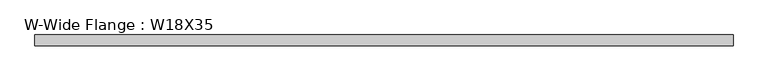
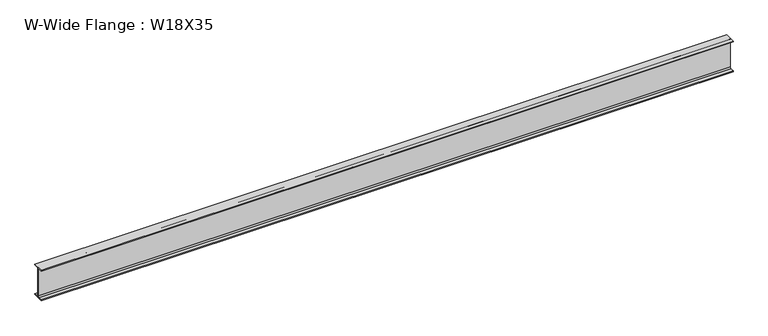
"""IFC4 building model written with IfcOpenShell, lengths in millimetres: beam geometry, W-Wide Flange : W18X35."""

from ifc_helpers import new_model, si_unit, point, frame, frame_2d, origin, place, context, project, spatial, polyline, circle_curve, trimmed, segment, composite_curve, outline, extrude, source, transform, mapped, element, save


def w_wide_flange_w18x35_eb31aa4e(model_context):
    return source(origin(), model_context, "Body", "SweptSolid", [
        extrude(outline(composite_curve([segment(polyline([(76.2, -213.995), (76.2, -224.79), (-76.2, -224.79), (-76.2, -213.995), (-21.59, -213.995)]), True, "CONTINUOUS"), segment(trimmed(circle_curve(frame_2d((-21.59, -196.215)), 17.78), [point((-21.59, -213.995))], [point((-3.81, -196.215))], True, "CARTESIAN"), True, "CONTINUOUS"), segment(polyline([(-3.81, -196.215), (-3.81, 196.215)]), True, "CONTINUOUS"), segment(trimmed(circle_curve(frame_2d((-21.59, 196.215)), 17.78), [point((-3.81, 196.215))], [point((-21.59, 213.995))], True, "CARTESIAN"), True, "CONTINUOUS"), segment(polyline([(-21.59, 213.995), (-76.2, 213.995), (-76.2, 224.79), (76.2, 224.79), (76.2, 213.995), (21.59, 213.995)]), True, "CONTINUOUS"), segment(trimmed(circle_curve(frame_2d((21.59, 196.215)), 17.78), [point((21.59, 213.995))], [point((3.81, 196.215))], True, "CARTESIAN"), True, "CONTINUOUS"), segment(polyline([(3.81, 196.215), (3.81, -196.215)]), True, "CONTINUOUS"), segment(trimmed(circle_curve(frame_2d((21.59, -196.215)), 17.78), [point((3.81, -196.215))], [point((21.59, -213.995))], True, "CARTESIAN"), True, "CONTINUOUS"), segment(polyline([(21.59, -213.995), (76.2, -213.995)]), True, "CONTINUOUS")], self_intersect=False)), frame((-4806.95, 0.0, 0.0), z_axis=(1.0, 0.0, 0.0), x_axis=(0.0, 1.0, 0.0)), (0.0, 0.0, 1.0), 9683.75),
    ])


if __name__ == "__main__":
    model = new_model("IFC4")
    model_context = context("Model", 3, world=origin())
    ifc_project = project(units=[si_unit("LENGTHUNIT", "METRE", prefix="MILLI")], contexts=[model_context])
    site = spatial("IfcSite", under=ifc_project)
    building = spatial("IfcBuilding", under=site)
    placement = place(None, origin())
    w_wide_flange_w18x35_shape = w_wide_flange_w18x35_eb31aa4e(model_context)
    element("IfcBeam", 1, ObjectType="W-Wide Flange : W18X35", at=placement, inside=building, context=model_context, shape_type="MappedRepresentation", body=[
        mapped(w_wide_flange_w18x35_shape, transform((0.0, 0.0, 0.0), x_axis=(1.0, 0.0, 0.0), y_axis=(0.0, 1.0, 0.0), z_axis=(0.0, 0.0, 1.0))),
    ])
    save(model, "model.ifc")

# Revit data of these elements
# Type "W-Wide Flange : W18X35"
#   Assembly Code = "B10"
#   W = 35
#   Length [instance default] = 5' - 0"
#   bf = 0' - 6"
#   d = 1' - 5.7"
#   k = 0' - 1 1/8"
#   k2 = 0' - 0.7"
#   tf = 0' - 0.425"
#   tw = 0' - 0.3"
#   A = 0.0715278 SF
#   Structural Material [instance default] = Steel ASTM A992
# Element 1 (IfcBeam, "W-Wide Flange : W18X35")
#   Structural Material = Steel ASTM A36
#   Materials on its faces: "Steel ASTM A36"
# Materials
#   "Steel ASTM A992": class "Metal", colour RGB 199 199 199, transparency 0, Description = "Structural steel 50ksi", Cost = 0
#   "Steel ASTM A36": class "Metal", colour RGB 199 199 199, transparency 0, Description = "Structural steel, ASTM A36 Grade B, mill finish", Cost = 0
